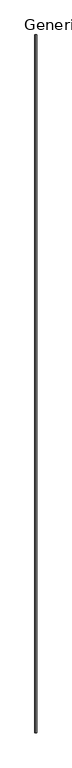
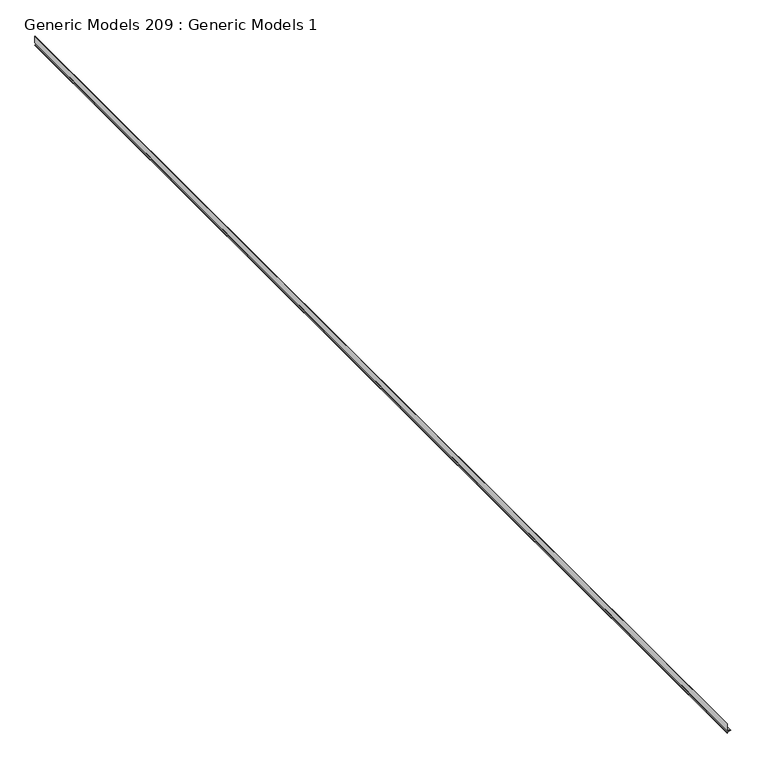
"""IFC4 building model written with IfcOpenShell, lengths in millimetres: proxy geometry, Generic Models 209 : Generic Models 1."""

from ifc_helpers import new_model, si_unit, frame, origin, place, context, project, spatial, polyline, outline, extrude, source, transform, mapped, element, save


def generic_models_209_generic_models_1_4a2ab0c1(model_context):
    return source(origin(), model_context, "Body", "SweptSolid", [
        extrude(outline(polyline([(126801.3526945, -8139.6830045), (126808.0882303, -8160.6380045), (126852.1526945, -8160.6380045), (126852.1526945, -8161.9080045), (126807.162451, -8161.9080045), (126801.3526945, -8143.8332068), (126795.8525366, -8160.9448095), (126790.7377862, -8161.9080045), (126790.5027546, -8160.659942), (126794.8747464, -8159.8366211), (126801.3526945, -8139.6830045)])), frame((0.0, -464.1230338, 0.0), z_axis=(0.0, 1.0, 0.0), x_axis=(0.0, 0.0, 1.0)), (0.0, 0.0, 1.0), 7518.4),
    ])


if __name__ == "__main__":
    model = new_model("IFC4")
    model_context = context("Model", 3, world=origin())
    ifc_project = project(units=[si_unit("LENGTHUNIT", "METRE", prefix="MILLI")], contexts=[model_context])
    site = spatial("IfcSite", under=ifc_project)
    building = spatial("IfcBuilding", under=site)
    placement = place(None, origin())
    generic_models_209_generic_models_1_shape = generic_models_209_generic_models_1_4a2ab0c1(model_context)
    element("IfcBuildingElementProxy", 1, Name="Generic Models 209 : Generic Models 1", ObjectType="Generic Models 209 : Generic Models 1", at=placement, inside=building, context=model_context, shape_type="MappedRepresentation", body=[
        mapped(generic_models_209_generic_models_1_shape, transform((0.0, 0.0, 0.0), x_axis=(1.0, 0.0, 0.0), y_axis=(0.0, 1.0, 0.0), z_axis=(0.0, 0.0, 1.0))),
    ])
    save(model, "model.ifc")

# Revit data of these elements
# Element 1 (IfcBuildingElementProxy, "Generic Models 209 : Generic Models 1")
#   Materials on its faces: "_ 16 GA. COPPER VENTED T REVEAL BEAD (CONT. AROUND PERIMETER OF BEAM)"
# Materials
#   "_ 16 GA. COPPER VENTED T REVEAL BEAD (CONT. AROUND PERIMETER OF BEAM)": class "Generic", colour RGB 253 192 103, transparency 0, Cost = 0
